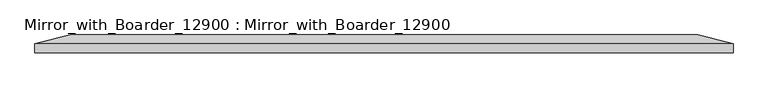
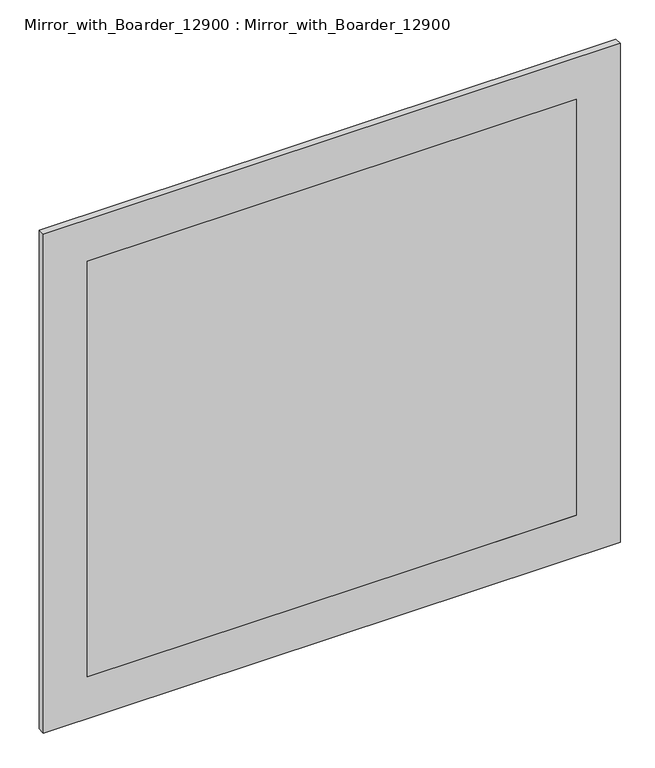
"""IFC4 building model written with IfcOpenShell, lengths in millimetres: proxy geometry, Mirror_with_Boarder_12900 : Mirror_with_Boarder_12900."""

from ifc_helpers import new_model, si_unit, frame, origin, place, context, project, spatial, polyline, outline, extrude, faceted_brep, source, transform, mapped, element, save


def mirror_with_boarder_12900_mirror_with_boarder_12900_c07f3b3f(model_context):
    return source(origin(), model_context, "Body", "SolidModel", [
        faceted_brep([(412.7003906, 63.9960938, 1027.1125), (-412.7003906, 63.9960938, 1027.1125), (-412.7003906, 63.9960938, 1766.8875), (412.7003906, 63.9960938, 1766.8875), (423.8128906, 59.2335938, 1016.0), (423.8128906, 59.2335938, 1778.0), (-423.8128906, 59.2335938, 1778.0), (-423.8128906, 59.2335938, 1016.0), (-423.8128906, 62.4085938, 1016.0), (423.8128906, 62.4085937, 1016.0), (-423.8128906, 62.4085938, 1778.0), (423.8128906, 62.4085937, 1778.0)], [[[0, 1, 2, 3]], [[4, 5, 6, 7]], [[4, 7, 8, 9]], [[7, 6, 10, 8]], [[6, 5, 11, 10]], [[5, 4, 9, 11]], [[8, 1, 0, 9]], [[1, 8, 10, 2]], [[2, 10, 11, 3]], [[9, 0, 3, 11]]]),
        extrude(outline(polyline([(-423.8128906, 59.2335938), (423.8128906, 59.2335938), (423.8128906, 50.8), (-423.8128906, 50.8), (-423.8128906, 59.2335938)])), frame((0.0, 0.0, 1016.0), z_axis=(0.0, 0.0, 1.0), x_axis=(1.0, 0.0, 0.0)), (0.0, 0.0, 1.0), 762.0),
        faceted_brep([(449.2128906, 76.2, 1803.4), (449.2128906, 76.2, 990.6), (-449.2128906, 76.2, 990.6), (-449.2128906, 76.2, 1803.4), (-423.8128906, 76.2, 1778.0), (-423.8128906, 76.2, 1016.0), (423.8128906, 76.2, 1016.0), (423.8128906, 76.2, 1778.0), (-500.0128906, 50.8, 1854.2), (-500.0128906, 50.8, 939.8), (500.0128906, 50.8, 939.8), (500.0128906, 50.8, 1854.2), (-423.8128906, 50.8, 1778.0), (423.8128906, 50.8, 1778.0), (423.8128906, 50.8, 1016.0), (-423.8128906, 50.8, 1016.0), (-423.8128906, 63.9960938, 1778.0), (-423.8128906, 62.4085937, 1778.0), (-423.8128906, 62.4085938, 1016.0), (-423.8128906, 63.9960938, 1016.0), (423.8128906, 62.4085938, 1016.0), (423.8128906, 63.9960938, 1016.0), (423.8128906, 62.4085937, 1778.0), (423.8128906, 63.9960938, 1778.0), (500.0128906, 63.5, 1854.2), (-500.0128906, 63.5, 1854.2), (500.0128906, 63.5, 939.8), (-500.0128906, 63.5, 939.8)], [[[0, 1, 2, 3], [4, 5, 6, 7]], [[8, 9, 10, 11], [12, 13, 14, 15]], [[5, 4, 16, 17, 12, 15, 18, 19]], [[6, 5, 19, 18, 15, 14, 20, 21]], [[7, 6, 21, 20, 14, 13, 22, 23]], [[4, 7, 23, 22, 13, 12, 17, 16]], [[8, 11, 24, 25]], [[11, 10, 26, 24]], [[10, 9, 27, 26]], [[9, 8, 25, 27]], [[26, 1, 0, 24]], [[1, 26, 27, 2]], [[2, 27, 25, 3]], [[24, 0, 3, 25]]]),
    ])


if __name__ == "__main__":
    model = new_model("IFC4")
    model_context = context("Model", 3, world=origin())
    ifc_project = project(units=[si_unit("LENGTHUNIT", "METRE", prefix="MILLI")], contexts=[model_context])
    site = spatial("IfcSite", under=ifc_project)
    building = spatial("IfcBuilding", under=site)
    placement = place(None, origin())
    mirror_with_boarder_12900_mirror_with_boarder_12900_shape = mirror_with_boarder_12900_mirror_with_boarder_12900_c07f3b3f(model_context)
    element("IfcBuildingElementProxy", 1, Name="Mirror_with_Boarder_12900 : Mirror_with_Boarder_12900", ObjectType="Mirror_with_Boarder_12900 : Mirror_with_Boarder_12900", at=placement, inside=building, context=model_context, shape_type="MappedRepresentation", body=[
        mapped(mirror_with_boarder_12900_mirror_with_boarder_12900_shape, transform((0.0, 0.0, 0.0), x_axis=(1.0, 0.0, 0.0), y_axis=(0.0, 1.0, 0.0), z_axis=(0.0, 0.0, 1.0))),
    ])
    save(model, "model.ifc")

# Revit data of these elements
# Type "Mirror_with_Boarder_12900 : Mirror_with_Boarder_12900"
#   Width = 3' - 3 95/256"
#   Height = 3' - 0"
#   Mirror Frame = Mirror Frame
#   Mirror = Mirror
#   Default Elevation = 0
# Element 1 (IfcBuildingElementProxy, "Mirror_with_Boarder_12900 : Mirror_with_Boarder_12900")
#   Materials on its faces: "Mirror Frame", "Mirror"
# Materials
#   "Mirror Frame": class "Miscellaneous", colour RGB 27 25 23, transparency 0
#   "Mirror": class "Glass", colour RGB 178 191 178, transparency 0, Cost = 0
